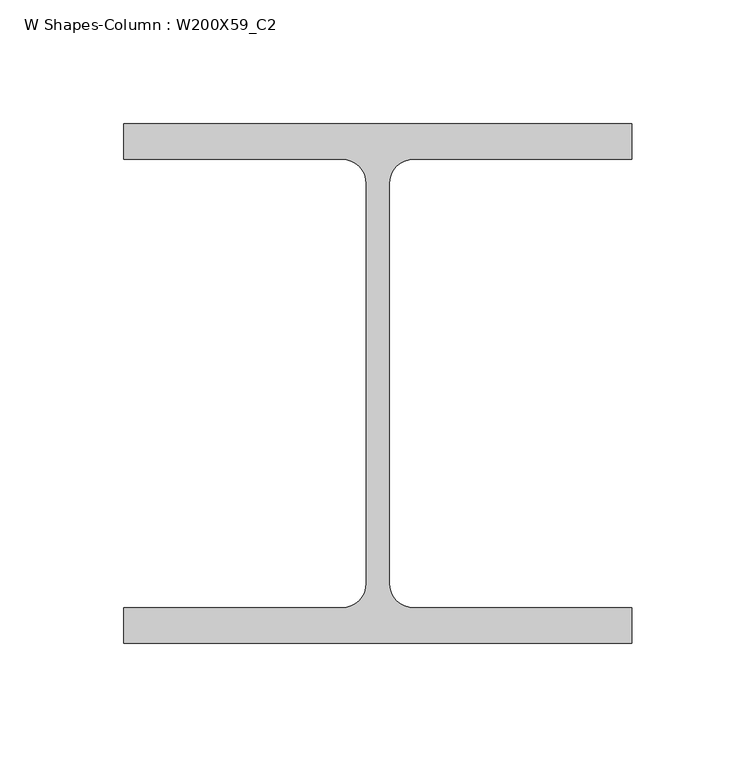
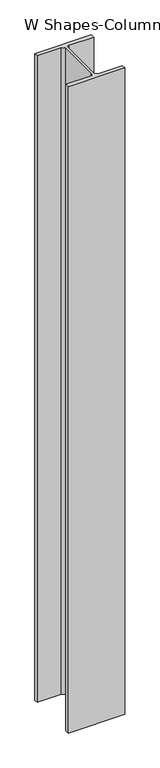
"""IFC4 building model written with IfcOpenShell, lengths in millimetres: column geometry, W Shapes-Column : W200X59_C2."""

from ifc_helpers import new_model, si_unit, point, frame, frame_2d, origin, place, context, project, spatial, polyline, circle_curve, trimmed, segment, composite_curve, outline, extrude, source, transform, mapped, element, save


def w_shapes_column_w200x59_c2_2bfd83e9(model_context):
    return source(origin(), model_context, "Body", "SweptSolid", [
        extrude(outline(composite_curve([segment(polyline([(102.489, 104.775), (102.489, 90.551), (14.5796, 90.551)]), True, "CONTINUOUS"), segment(trimmed(circle_curve(frame_2d((14.5796, 80.5434)), 10.0076), [point((14.5796, 90.551))], [point((4.572, 80.5434))], True, "CARTESIAN"), True, "CONTINUOUS"), segment(polyline([(4.572, 80.5434), (4.572, -80.5434)]), True, "CONTINUOUS"), segment(trimmed(circle_curve(frame_2d((14.5796, -80.5434)), 10.0076), [point((4.572, -80.5434))], [point((14.5796, -90.551))], True, "CARTESIAN"), True, "CONTINUOUS"), segment(polyline([(14.5796, -90.551), (102.489, -90.551), (102.489, -104.775), (-102.489, -104.775), (-102.489, -90.551), (-14.5796, -90.551)]), True, "CONTINUOUS"), segment(trimmed(circle_curve(frame_2d((-14.5796, -80.5434)), 10.0076), [point((-14.5796, -90.551))], [point((-4.572, -80.5434))], True, "CARTESIAN"), True, "CONTINUOUS"), segment(polyline([(-4.572, -80.5434), (-4.572, 80.5434)]), True, "CONTINUOUS"), segment(trimmed(circle_curve(frame_2d((-14.5796, 80.5434)), 10.0076), [point((-4.572, 80.5434))], [point((-14.5796, 90.551))], True, "CARTESIAN"), True, "CONTINUOUS"), segment(polyline([(-14.5796, 90.551), (-102.489, 90.551), (-102.489, 104.775), (102.489, 104.775)]), True, "CONTINUOUS")], self_intersect=False)), frame((0.0, 0.0, 3526.0), z_axis=(0.0, 0.0, 1.0), x_axis=(1.0, 0.0, 0.0)), (0.0, 0.0, 1.0), 2484.0),
    ])


if __name__ == "__main__":
    model = new_model("IFC4")
    model_context = context("Model", 3, world=origin())
    ifc_project = project(units=[si_unit("LENGTHUNIT", "METRE", prefix="MILLI")], contexts=[model_context])
    site = spatial("IfcSite", under=ifc_project)
    building = spatial("IfcBuilding", under=site)
    placement = place(None, origin())
    w_shapes_column_w200x59_c2_shape = w_shapes_column_w200x59_c2_2bfd83e9(model_context)
    element("IfcColumn", 1, ObjectType="W Shapes-Column : W200X59_C2", at=placement, inside=building, context=model_context, shape_type="MappedRepresentation", body=[
        mapped(w_shapes_column_w200x59_c2_shape, transform((0.0, 0.0, 0.0), x_axis=(1.0, 0.0, 0.0), y_axis=(0.0, 1.0, 0.0), z_axis=(0.0, 0.0, 1.0))),
    ])
    save(model, "model.ifc")

# Revit data of these elements
# Type "W Shapes-Column : W200X59_C2"
#   Section Name Key = "W8x40"
#   Assembly Code = "B10"
#   Width = 20.4978 cm
#   Web Thickness = 0.9144 cm
#   Web Fillet = 1.0008 cm
#   Warping Constant = 194957.0 cm⁶
#   Torsional Moment of Inertia = 46.6179 cm⁴
#   Section Area = 75.4837 cm²
#   Plastic Modulus weak axis = 303.161 cm³
#   Plastic Modulus strong axis = 652.205 cm³
#   Perimeter = 1.20396 m²/m
#   Nominal Weight = 59.5266 kgf/m
#   Moment of Inertia weak axis = 2043.70 cm⁴
#   Moment of Inertia strong axis = 6076.98 cm⁴
#   Height = 20.955 cm
#   Flange Thickness = 1.4224 cm
#   Elastic Modulus weak axis = 199.922 cm³
#   Elastic Modulus strong axis = 581.741 cm³
#   Clear Web Height = 19.05 cm
#   Centroid Vertical = 10.4775 cm
#   Centroid Horizontal = 10.2489 cm
#   Bolt Spacing = 13.97 cm
#   Structural Material [instance default] = Steel ASTM A992
#   Principal Axes Angle = 0
# Element 1 (IfcColumn, "W Shapes-Column : W200X59_C2")
#   Structural Material = none
# Materials
#   "Steel ASTM A992": class "Metal", colour RGB 199 199 199, transparency 0, Description = "Structural steel 50ksi", Cost = 0
